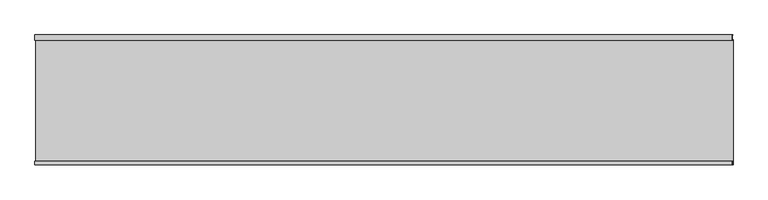
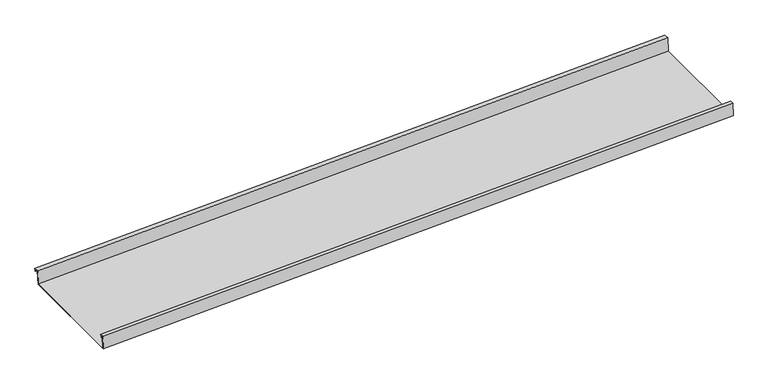
"""IFC4 building model written with IfcOpenShell, lengths in millimetres: proxy geometry, Generic Models 2:Generic Models 2:310765:Generic Models 2:310765 : Generic Models 2:Generic Models 2:310765:78 : Generic Models 2:Generic Models 2:310765:Generic Models 2:310765 : Generic Models 2:Generic Models 2:310765:300385."""

from ifc_helpers import new_model, si_unit, frame, origin, place, context, project, spatial, polyline, outline, extrude, source, transform, mapped, element, save


def generic_models_8ed0f672(model_context):
    return source(origin(), model_context, "Body", "SweptSolid", [
        extrude(outline(polyline([(1.5875, 0.0), (1.5875, 50.8), (407.9875, 50.8), (407.9875, 1.5874999), (396.875, 1.5874999), (396.875, 11.1125), (398.4625, 11.1125), (398.4625, 3.175), (406.4, 3.175), (406.4, 49.2124999), (3.175, 49.2124999), (3.175, -1.5875), (-14.2875, -1.5875), (-14.2875, 9.525), (-12.7, 9.525), (-12.7, 0.0), (1.5875, 0.0)])), frame((558060.6329583, -578114.072634, 3904.6995643), z_axis=(0.9991330730923568, 0.0, 0.041630544712067834), x_axis=(0.0, -1.0, 0.0)), (0.0, 0.0, 1.0), 2268.8048169),
    ])


if __name__ == "__main__":
    model = new_model("IFC4")
    model_context = context("Model", 3, world=origin())
    ifc_project = project(units=[si_unit("LENGTHUNIT", "METRE", prefix="MILLI")], contexts=[model_context])
    site = spatial("IfcSite", under=ifc_project)
    building = spatial("IfcBuilding", under=site)
    placement = place(None, origin())
    generic_models_shape = generic_models_8ed0f672(model_context)
    element("IfcBuildingElementProxy", 1, Name="Generic Models 2:Generic Models 2:310765:Generic Models 2:310765 : Generic Models 2:Generic Models 2:310765:78 : Generic Models 2:Generic Models 2:310765:Generic Models 2:310765 : Generic Models 2:Generic Models 2:310765:300385", ObjectType="Generic Models 2:Generic Models 2:310765:Generic Models 2:310765 : Generic Models 2:Generic Models 2:310765:78 : Generic Models 2:Generic Models 2:310765:Generic Models 2:310765 : Generic Models 2:Generic Models 2:310765:300385", at=placement, inside=building, context=model_context, shape_type="MappedRepresentation", body=[
        mapped(generic_models_shape, transform((0.0, 0.0, 0.0), x_axis=(1.0, 0.0, 0.0), y_axis=(0.0, 1.0, 0.0), z_axis=(0.0, 0.0, 1.0))),
    ])
    save(model, "model.ifc")

# Revit data of these elements
# Type "Generic Models 2:Generic Models 2:310765:Generic Models 2:310765 : Generic Models 2:Generic Models 2:310765:78 : Generic Models 2:Generic Models 2:310765:Generic Models 2:310765 : Generic Models 2:Generic Models 2:310765:300385"
#   NameOverride = "Generic Models 2:Generic Models 2:310765:Generic Models 2:310765 : Generic Models 2:Generic Models 2:310765:300385"
#   ObjectTypeOverride = "Generic Models 2:310765 : Generic Models 2:Generic Models 2:310765"
#   Reference = "Generic Models 2"
#   Tag = "300385"
# Element 1 (IfcBuildingElementProxy, "Generic Models 2:Generic Models 2:310765:Generic Models 2:310765 : Generic Models 2:Generic Models 2:310765:78 : Generic Models 2:Generic Models 2:310765:Generic Models 2:310765 : Generic Models 2:Generic Models 2:310765:300385")
#   Materials on its faces: "STRUCTURAL STANDING SEAM SHEET METAL ROOFING - BATTENLOK - COLOR T.B.D."
# Materials
#   "STRUCTURAL STANDING SEAM SHEET METAL ROOFING - BATTENLOK - COLOR T.B.D.": class "Generic", colour RGB 120 120 120, transparency 0, Cost = 0
